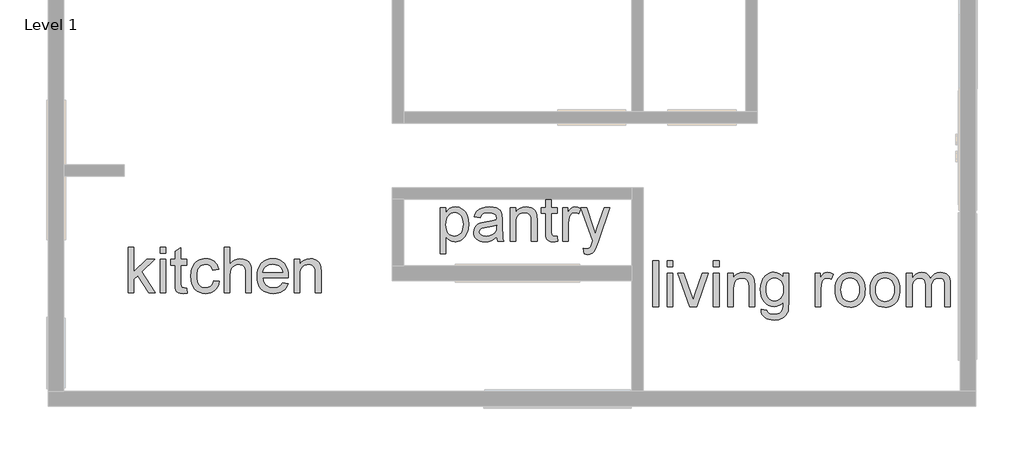
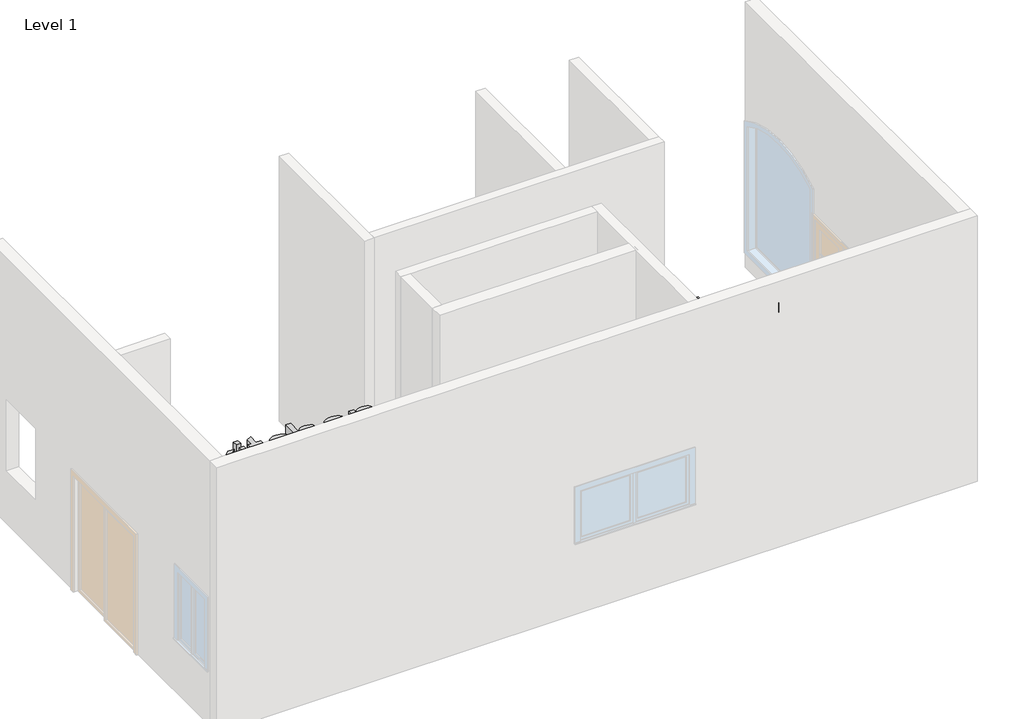
# One storey, part 2 of 3: 3 proxies.
"""IFC4 building model written with IfcOpenShell, lengths in millimetres."""

from ifc_helpers import new_model, si_unit, origin, origin_with_axes, place, context, project, spatial, polyline, outline, extrude, element, save

model = new_model("IFC4")

# Units and contexts
model_context = context("Model", 3, world=origin())
ifc_project = project(units=[si_unit("LENGTHUNIT", "METRE", prefix="MILLI")], contexts=[model_context])

# Site, building, storey
site = spatial("IfcSite", under=ifc_project)
building = spatial("IfcBuilding", under=site)
storey = spatial("IfcBuildingStorey", under=building, Name="Level 1", Elevation=0.0)

# Proxies
placement = place(None, origin())
element("IfcBuildingElementProxy", 1, Name="24\" Arial", ObjectType="24\" Arial", at=placement, inside=storey, context=model_context, shape_type="SweptSolid", body=[
    extrude(outline(polyline([(-2541.0046278, -2163.6481943), (-2541.0046278, -1554.5140062), (-2464.8628543, -1554.5140062), (-2464.8628543, -1881.8344036), (-2294.1387215, -1716.3152749), (-2188.8489253, -1716.3152749), (-2361.6550597, -1883.9164053), (-2179.3312036, -2163.6481943), (-2268.2624157, -2163.6481943), (-2416.2332451, -1936.8587322), (-2464.8628543, -1984.0011974), (-2464.8628543, -2163.6481943), (-2541.0046278, -2163.6481943)])), origin_with_axes(), (0.0, 0.0, 1.0), 152.4),
    extrude(outline(polyline([(-2112.7071518, -2163.6481943), (-2112.7071518, -1716.3152749), (-2036.5653783, -1716.3152749), (-2036.5653783, -2163.6481943), (-2112.7071518, -2163.6481943)])), origin_with_axes(), (0.0, 0.0, 1.0), 152.4),
    extrude(outline(polyline([(-2112.7071518, -1630.6557797), (-2112.7071518, -1554.5140062), (-2036.5653783, -1554.5140062), (-2036.5653783, -1630.6557797), (-2112.7071518, -1630.6557797)])), origin_with_axes(), (0.0, 0.0, 1.0), 152.4),
    extrude(outline(polyline([(-1760.5514493, -2100.1471449), (-1751.0337276, -2165.8789103), (-1781.1855725, -2171.3441646), (-1807.9913433, -2173.165916), (-1844.5379075, -2170.005735), (-1871.7898215, -2160.5251919), (-1891.0483365, -2145.9140019), (-1903.6147034, -2127.3618803), (-1910.5299231, -2095.4998198), (-1912.8349963, -2040.9588131), (-1912.8349963, -1792.4570484), (-1969.9413265, -1792.4570484), (-1969.9413265, -1716.3152749), (-1912.8349963, -1716.3152749), (-1912.8349963, -1607.6050475), (-1836.6932228, -1562.8420126), (-1836.6932228, -1716.3152749), (-1760.5514493, -1716.3152749), (-1760.5514493, -1792.4570484), (-1836.6932228, -1792.4570484), (-1836.6932228, -2038.7280971), (-1832.677934, -2077.9886991), (-1819.6654238, -2091.8934956), (-1808.6791474, -2095.7414808), (-1793.7147608, -2097.0241425), (-1760.5514493, -2100.1471449)])), origin_with_axes(), (0.0, 0.0, 1.0), 152.4),
    extrude(outline(polyline([(-1398.8780251, -2001.8469256), (-1322.7362516, -2011.3646473), (-1331.0177848, -2047.2931172), (-1343.9652324, -2079.0854678), (-1361.5785943, -2106.7416991), (-1383.8578705, -2130.2618112), (-1409.8643015, -2149.032357), (-1438.6591274, -2162.4398898), (-1470.2423484, -2170.4844094), (-1504.6139645, -2173.165916), (-1547.3182343, -2169.4248193), (-1585.6075453, -2158.2015293), (-1619.4818976, -2139.496046), (-1648.941291, -2113.3083694), (-1672.7867158, -2080.1311159), (-1689.8191621, -2040.456902), (-1700.0386299, -1994.2857277), (-1703.4451191, -1941.617593), (-1697.6266682, -1873.8595939), (-1690.3536045, -1843.3684943), (-1680.1713153, -1815.1359946), (-1667.0100908, -1789.7290686), (-1650.800221, -1767.7146899), (-1631.5417061, -1749.0928584), (-1609.2345459, -1733.8635742), (-1584.88721, -1722.02219), (-1559.5081679, -1713.5640585), (-1533.0974197, -1708.4891795), (-1505.6549653, -1706.7975532), (-1471.8735595, -1709.1212157), (-1441.3173974, -1716.0922033), (-1413.9864788, -1727.7105159), (-1389.8808038, -1743.9761535), (-1369.409337, -1764.5173302), (-1352.9810429, -1788.96226), (-1340.5959217, -1817.3109427), (-1332.2539732, -1849.5633785), (-1408.3957468, -1859.0811002), (-1422.2075968, -1825.8620208), (-1443.7154171, -1802.0491273), (-1471.7294925, -1787.7167769), (-1505.0601077, -1782.9393267), (-1530.9317662, -1785.2908732), (-1554.2659852, -1792.3455126), (-1575.0627648, -1804.103245), (-1593.3221049, -1820.5640703), (-1608.1888977, -1842.1090692), (-1618.8080354, -1869.1193223), (-1625.1795181, -1901.5948297), (-1627.3033456, -1939.5355914), (-1625.2259913, -1978.047974), (-1618.9939284, -2010.8999148), (-1608.607157, -2038.0914136), (-1594.0656769, -2059.6224705), (-1576.1688282, -2075.985702), (-1555.7159507, -2087.6737245), (-1532.7070444, -2094.686538), (-1507.1421093, -2097.0241425), (-1467.7142036, -2091.1871022), (-1450.663168, -2083.8908019), (-1435.3874106, -2073.6759814), (-1422.3144853, -2060.4311051), (-1411.8719459, -2044.044637), (-1404.0597925, -2024.5165771), (-1398.8780251, -2001.8469256)])), origin_with_axes(), (0.0, 0.0, 1.0), 152.4),
    extrude(outline(polyline([(-1256.1121997, -2163.6481943), (-1256.1121997, -1554.5140062), (-1179.9704262, -1554.5140062), (-1179.9704262, -1778.4778947), (-1152.0028241, -1747.1177453), (-1120.5962015, -1724.7176386), (-1085.7505583, -1711.2775745), (-1047.4658946, -1706.7975532), (-1001.4759659, -1711.6865391), (-961.9551138, -1726.353497), (-930.8366253, -1749.6458901), (-919.1532501, -1764.0944237), (-910.0537877, -1780.4111819), (-898.3425286, -1822.6832505), (-894.4387755, -1880.495974), (-894.4387755, -2163.6481943), (-970.580549, -2163.6481943), (-970.580549, -1888.3778373), (-972.095577, -1862.6688352), (-976.6406609, -1840.7148717), (-984.2158007, -1822.5159468), (-994.8209965, -1808.0720605), (-1008.2052926, -1797.0764895), (-1024.1177335, -1789.2225102), (-1042.5583193, -1784.5101226), (-1063.5270499, -1782.9393267), (-1095.7051285, -1787.1776871), (-1125.9127413, -1799.8927685), (-1150.9339393, -1819.8576769), (-1167.5527737, -1845.8455185), (-1176.8660131, -1880.3844382), (-1179.9704262, -1926.0025809), (-1179.9704262, -2163.6481943), (-1256.1121997, -2163.6481943)])), origin_with_axes(), (0.0, 0.0, 1.0), 152.4),
    extrude(outline(polyline([(-476.5513076, -2030.4000906), (-401.8966781, -2039.9178123), (-413.3430397, -2069.8187017), (-428.7953954, -2096.1690347), (-448.2537454, -2118.9688113), (-471.7180895, -2138.2180317), (-498.946767, -2153.507731), (-529.6981168, -2164.4289449), (-563.972139, -2170.9816732), (-601.7688336, -2173.165916), (-649.01354, -2169.3969354), (-691.1090102, -2158.0899935), (-728.0552443, -2139.2450905), (-759.8522423, -2112.8622262), (-785.4218246, -2079.6756781), (-803.6858121, -2040.4197234), (-814.6442045, -1995.0943623), (-818.297002, -1943.6995946), (-814.6070259, -1890.5620801), (-803.5370977, -1843.7263383), (-785.0872172, -1803.1923692), (-759.2573847, -1768.960173), (-727.5440386, -1741.7640268), (-691.4436176, -1722.3382081), (-650.9561218, -1710.6827169), (-606.0815512, -1706.7975532), (-562.6522987, -1710.6734223), (-523.3777547, -1722.3010295), (-488.2579194, -1741.680375), (-457.2927926, -1768.8114586), (-432.0159917, -1802.9692976), (-413.9611339, -1843.4289095), (-403.1282192, -1890.1902941), (-399.5172477, -1943.2534514), (-399.9633909, -1963.7760388), (-742.1552285, -1963.7760388), (-737.744917, -1994.1602499), (-728.9754147, -2020.7708331), (-715.8467214, -2043.6077884), (-698.3588373, -2062.6711157), (-677.4784059, -2077.7005649), (-654.1720708, -2088.4358858), (-628.439832, -2094.8770783), (-600.2816896, -2097.0241425), (-559.7570152, -2093.0460322), (-525.6270601, -2081.1117015), (-497.8918242, -2060.4775783), (-476.5513076, -2030.4000906)]), holes=[polyline([(-742.1552285, -1887.6342653), (-475.6590212, -1887.6342653), (-485.9574935, -1847.4070197), (-494.815295, -1831.5875253), (-506.1454735, -1818.630783), (-526.9097218, -1803.0157709), (-550.5367223, -1791.8621908), (-577.026475, -1785.1700427), (-606.37898, -1782.9393267), (-633.1522196, -1784.7192522), (-657.7040378, -1790.0590287), (-680.0344346, -1798.9586561), (-700.1434101, -1811.4181346), (-717.0178473, -1826.8611957), (-729.6446295, -1844.7115712), (-738.0237565, -1864.9692611), (-742.1552285, -1887.6342653)])]), origin_with_axes(), (0.0, 0.0, 1.0), 152.4),
    extrude(outline(polyline([(-323.3754741, -2163.6481943), (-323.3754741, -1716.3152749), (-247.2337006, -1716.3152749), (-247.2337006, -1778.7753235), (-220.7811265, -1747.285049), (-189.0120125, -1724.7919958), (-151.9263586, -1711.2961638), (-109.5241649, -1706.7975532), (-71.9923679, -1710.4224667), (-37.6207519, -1721.2972073), (-8.956051, -1738.0647561), (11.4550006, -1759.3680941), (25.3040292, -1785.1514534), (34.2826612, -1815.3590662), (38.2979501, -1888.9726949), (38.2979501, -2163.6481943), (-37.8438235, -2163.6481943), (-37.8438235, -1899.2339886), (-40.0373609, -1859.8618508), (-46.6179731, -1831.8663648), (-58.7567862, -1811.8085099), (-77.6249258, -1796.2492656), (-101.8096054, -1786.2668114), (-129.8980379, -1782.9393267), (-153.01848, -1784.8075514), (-174.493769, -1790.4122254), (-194.323905, -1799.7533487), (-212.5088879, -1812.8309214), (-227.7009935, -1831.1320874), (-238.5524974, -1856.1439908), (-245.0633998, -1887.8666315), (-247.2337006, -1926.3000097), (-247.2337006, -2163.6481943), (-323.3754741, -2163.6481943)])), origin_with_axes(), (0.0, 0.0, 1.0), 152.4),
])
element("IfcBuildingElementProxy", 2, Name="24\" Arial", ObjectType="24\" Arial", at=placement, inside=storey, context=model_context, shape_type="SweptSolid", body=[
    extrude(outline(polyline([(1631.9732742, -1642.5079695), (1631.9732742, -1023.8560597), (1708.1150477, -1023.8560597), (1708.1150477, -1098.5106892), (1732.9503528, -1061.6852856), (1760.7599458, -1035.3814258), (1793.1796853, -1019.59911), (1831.8454297, -1014.338338), (1858.400245, -1016.1786787), (1883.3377912, -1021.6997009), (1906.6580682, -1030.9014045), (1928.3610762, -1043.7837895), (1947.9727879, -1060.0122485), (1965.0191761, -1079.2521742), (1979.500241, -1101.5035665), (1991.4159824, -1126.7664255), (2007.3656019, -1182.8689334), (2012.6821418, -1244.1020882), (2006.6777978, -1309.2204067), (1999.1723679, -1339.2003005), (1988.664766, -1367.4606841), (1975.2990591, -1393.2626328), (1959.2193145, -1415.8672218), (1940.425532, -1435.2744512), (1918.9177117, -1451.4843209), (1895.7507964, -1464.2691121), (1871.9797288, -1473.4011058), (1847.6045089, -1478.8803021), (1822.6251368, -1480.7067008), (1787.6214846, -1475.8177149), (1756.372871, -1461.150757), (1729.622868, -1439.0109005), (1708.1150477, -1411.7032185), (1708.1150477, -1642.5079695), (1631.9732742, -1642.5079695)]), holes=[polyline([(1708.1150477, -1251.091665), (1710.1738127, -1287.7869436), (1716.3501077, -1319.3515753), (1726.6439327, -1345.7855601), (1741.0552876, -1367.0888981), (1758.403752, -1383.4846609), (1777.5089053, -1395.19592), (1798.3707474, -1402.2226755), (1820.9892784, -1404.5649273), (1843.9331221, -1402.1390236), (1865.1760449, -1394.8613126), (1884.7180467, -1382.7317942), (1902.5591275, -1365.7504685), (1917.4259204, -1343.6756746), (1928.0450581, -1316.2657514), (1934.4165407, -1283.5206992), (1936.5403683, -1245.4405178), (1934.4676613, -1209.0612573), (1928.2495404, -1177.5523935), (1917.8860055, -1150.9139264), (1903.3770568, -1129.1458559), (1885.9867664, -1112.2295927), (1866.979207, -1100.1465476), (1846.3543785, -1092.8967205), (1824.1122808, -1090.4801115), (1801.939893, -1093.0500823), (1781.0780509, -1100.7599945), (1761.5267544, -1113.6098483), (1743.2860036, -1131.5996435), (1727.8987104, -1154.4877193), (1716.9077867, -1182.0324149), (1710.3132325, -1214.2337301), (1708.1150477, -1251.091665)])]), origin_with_axes(), (0.0, 0.0, 1.0), 152.4),
    extrude(outline(polyline([(2383.8732877, -1414.082649), (2347.4940272, -1445.2754947), (2310.0365874, -1465.6865463), (2270.6458603, -1476.9516622), (2228.4667382, -1480.7067008), (2194.564502, -1478.4481008), (2164.8355637, -1471.6723009), (2139.2799233, -1460.3793011), (2117.8975808, -1444.5691013), (2101.0138489, -1425.2455237), (2088.9540404, -1403.4123907), (2081.7181553, -1379.0697021), (2079.3061936, -1352.217458), (2082.9496964, -1320.6528263), (2093.880205, -1291.9881254), (2110.7407002, -1267.4502492), (2132.1741633, -1248.2660914), (2157.362665, -1233.7664373), (2185.4882762, -1223.282072), (2251.368756, -1211.8310631), (2329.2207452, -1199.7851966), (2383.4271445, -1185.6573284), (2383.8732877, -1168.7038867), (2378.631105, -1134.7226459), (2372.0783767, -1122.1376897), (2362.9045571, -1112.4898429), (2347.047884, -1102.8605854), (2327.7336012, -1095.9825444), (2278.7322059, -1090.4801115), (2233.3743135, -1094.1422037), (2201.698146, -1105.1284801), (2180.0973792, -1125.4465852), (2164.9656888, -1157.1041633), (2088.8239153, -1147.5864417), (2102.0409077, -1105.9464093), (2121.7641552, -1073.229241), (2149.8339985, -1048.2080429), (2188.0907782, -1029.6559213), (2234.8800468, -1018.1677338), (2288.5473564, -1014.338338), (2340.0211286, -1017.7215906), (2380.8246425, -1027.8713485), (2411.5899342, -1043.133164), (2432.9490401, -1061.8525893), (2447.1140869, -1084.996268), (2456.2972012, -1113.5308437), (2460.0150612, -1180.1548956), (2460.0150612, -1274.8859693), (2463.8816356, -1407.1674293), (2469.6071401, -1439.8660083), (2479.0505046, -1471.1889791), (2402.9087311, -1471.1889791), (2390.7141501, -1444.7178157), (2383.8732877, -1414.082649)]), holes=[polyline([(2383.8732877, -1261.7991019), (2332.7155336, -1274.4770047), (2261.0351921, -1285.147263), (2195.5264983, -1297.4905583), (2178.48011, -1305.9301006), (2165.8579752, -1317.5670025), (2158.0504692, -1331.5089776), (2155.4479671, -1346.8637395), (2161.1177037, -1369.5055071), (2178.1269133, -1388.0576287), (2206.1038101, -1400.4381026), (2244.676608, -1404.5649273), (2285.5730684, -1400.0105487), (2321.7106679, -1386.3474131), (2351.007405, -1366.215201), (2371.381278, -1342.2535931), (2380.4156778, -1317.5670025), (2383.4271445, -1283.3626901), (2383.8732877, -1261.7991019)])]), origin_with_axes(), (0.0, 0.0, 1.0), 152.4),
    extrude(outline(polyline([(2564.7099998, -1471.1889791), (2564.7099998, -1023.8560597), (2640.8517733, -1023.8560597), (2640.8517733, -1086.3161083), (2667.3043475, -1054.8258338), (2699.0734615, -1032.3327806), (2736.1591153, -1018.8369486), (2778.561309, -1014.338338), (2816.0931061, -1017.9632515), (2850.4647221, -1028.8379921), (2879.1294229, -1045.6055409), (2899.5404745, -1066.9088789), (2913.3895032, -1092.6922382), (2922.3681352, -1122.899851), (2926.383424, -1196.5134797), (2926.383424, -1471.1889791), (2850.2416505, -1471.1889791), (2850.2416505, -1206.7747734), (2848.0481131, -1167.4026356), (2841.4675008, -1139.4071496), (2829.3286878, -1119.3492947), (2810.4605481, -1103.7900504), (2786.2758686, -1093.8075963), (2758.187436, -1090.4801115), (2735.0669939, -1092.3483362), (2713.5917049, -1097.9530102), (2693.7615689, -1107.2941335), (2675.576586, -1120.3717062), (2660.3844805, -1138.6728722), (2649.5329765, -1163.6847756), (2643.0220741, -1195.4074164), (2640.8517733, -1233.8407945), (2640.8517733, -1471.1889791), (2564.7099998, -1471.1889791)])), origin_with_axes(), (0.0, 0.0, 1.0), 152.4),
    extrude(outline(polyline([(3192.8796313, -1407.6879297), (3202.397353, -1473.4196951), (3172.2455081, -1478.8849494), (3145.4397373, -1480.7067008), (3108.8931731, -1477.5465198), (3081.6412591, -1468.0659767), (3062.3827441, -1453.4547867), (3049.8163772, -1434.9026652), (3042.9011575, -1403.0406047), (3040.5960843, -1348.499598), (3040.5960843, -1099.9978332), (2983.4897541, -1099.9978332), (2983.4897541, -1023.8560597), (3040.5960843, -1023.8560597), (3040.5960843, -915.1458323), (3116.7378578, -870.3827974), (3116.7378578, -1023.8560597), (3192.8796313, -1023.8560597), (3192.8796313, -1099.9978332), (3116.7378578, -1099.9978332), (3116.7378578, -1346.2688819), (3120.7531466, -1385.5294839), (3133.7656567, -1399.4342804), (3144.7519331, -1403.2822656), (3159.7163198, -1404.5649273), (3192.8796313, -1407.6879297)])), origin_with_axes(), (0.0, 0.0, 1.0), 152.4),
    extrude(outline(polyline([(3269.0214048, -1471.1889791), (3269.0214048, -1023.8560597), (3335.6454566, -1023.8560597), (3335.6454566, -1090.0339683), (3360.2576901, -1051.6656528), (3382.9366363, -1029.0610637), (3405.6899397, -1018.0190194), (3430.5252447, -1014.338338), (3468.4474171, -1020.2125569), (3506.9644471, -1037.8352134), (3481.5342844, -1106.0951237), (3454.7656922, -1094.3838646), (3427.9970999, -1090.4801115), (3405.2623858, -1094.2351502), (3384.9442807, -1105.5002661), (3368.5299287, -1123.4203514), (3357.5064737, -1147.1402985), (3348.2490022, -1189.6726173), (3345.1631783, -1236.0715105), (3345.1631783, -1471.1889791), (3269.0214048, -1471.1889791)])), origin_with_axes(), (0.0, 0.0, 1.0), 152.4),
    extrude(outline(polyline([(3554.5530555, -1642.5079695), (3545.0353338, -1569.1917696), (3583.7010782, -1575.8839177), (3604.0377726, -1573.7833268), (3619.8386777, -1567.481554), (3632.1447944, -1557.4247426), (3641.9971235, -1544.0590358), (3662.8171397, -1487.9937065), (3668.7657158, -1469.5531207), (3506.9644471, -1023.8560597), (3587.2702238, -1023.8560597), (3673.0784334, -1272.20911), (3702.9700281, -1371.5503302), (3732.8616228, -1283.8088333), (3821.0492628, -1023.8560597), (3900.760182, -1023.8560597), (3745.0562037, -1481.896416), (3704.6058865, -1581.2376361), (3683.8974061, -1612.9509822), (3660.4377093, -1634.923535), (3633.1857952, -1647.7501522), (3601.1006631, -1652.0256912), (3579.0537531, -1649.6462608), (3554.5530555, -1642.5079695)])), origin_with_axes(), (0.0, 0.0, 1.0), 152.4),
])
element("IfcBuildingElementProxy", 3, Name="24\" Arial", ObjectType="24\" Arial", at=placement, inside=storey, context=model_context, shape_type="SweptSolid", body=[
    extrude(outline(polyline([(4474.7005786, -2345.8743036), (4474.7005786, -1736.7401154), (4550.8423522, -1736.7401154), (4550.8423522, -2345.8743036), (4474.7005786, -2345.8743036)])), origin_with_axes(), (0.0, 0.0, 1.0), 152.4),
    extrude(outline(polyline([(4665.0550124, -2345.8743036), (4665.0550124, -1898.5413841), (4741.196786, -1898.5413841), (4741.196786, -2345.8743036), (4665.0550124, -2345.8743036)])), origin_with_axes(), (0.0, 0.0, 1.0), 152.4),
    extrude(outline(polyline([(4665.0550124, -1812.8818889), (4665.0550124, -1736.7401154), (4741.196786, -1736.7401154), (4741.196786, -1812.8818889), (4665.0550124, -1812.8818889)])), origin_with_axes(), (0.0, 0.0, 1.0), 152.4),
    extrude(outline(polyline([(4965.1606745, -2345.8743036), (4807.8208378, -1898.5413841), (4888.4240433, -1898.5413841), (4983.7499746, -2166.5247355), (5012.4518541, -2256.6456627), (5040.558876, -2171.5810251), (5136.4796649, -1898.5413841), (5217.0828704, -1898.5413841), (5061.676321, -2345.8743036), (4965.1606745, -2345.8743036)])), origin_with_axes(), (0.0, 0.0, 1.0), 152.4),
    extrude(outline(polyline([(5283.7069223, -2345.8743036), (5283.7069223, -1898.5413841), (5359.8486958, -1898.5413841), (5359.8486958, -2345.8743036), (5283.7069223, -2345.8743036)])), origin_with_axes(), (0.0, 0.0, 1.0), 152.4),
    extrude(outline(polyline([(5283.7069223, -1812.8818889), (5283.7069223, -1736.7401154), (5359.8486958, -1736.7401154), (5359.8486958, -1812.8818889), (5283.7069223, -1812.8818889)])), origin_with_axes(), (0.0, 0.0, 1.0), 152.4),
    extrude(outline(polyline([(5474.0613561, -2345.8743036), (5474.0613561, -1898.5413841), (5550.2031296, -1898.5413841), (5550.2031296, -1961.0014327), (5576.6557037, -1929.5111582), (5608.4248177, -1907.018105), (5645.5104716, -1893.5222731), (5687.9126653, -1889.0236624), (5725.4444623, -1892.648576), (5759.8160783, -1903.5233166), (5788.4807792, -1920.2908653), (5808.8918308, -1941.5942033), (5822.7408594, -1967.3775627), (5831.7194914, -1997.5851755), (5835.7347803, -2071.1988042), (5835.7347803, -2345.8743036), (5759.5930067, -2345.8743036), (5759.5930067, -2081.4600979), (5757.3994693, -2042.0879601), (5750.8188571, -2014.092474), (5738.680044, -1994.0346191), (5719.8119044, -1978.4753749), (5695.6272248, -1968.4929207), (5667.5387923, -1965.165436), (5644.4183502, -1967.0336606), (5622.9430612, -1972.6383346), (5603.1129252, -1981.979458), (5584.9279423, -1995.0570306), (5569.7358367, -2013.3581967), (5558.8843328, -2038.3701001), (5552.3734304, -2070.0927408), (5550.2031296, -2108.5261189), (5550.2031296, -2345.8743036), (5474.0613561, -2345.8743036)])), origin_with_axes(), (0.0, 0.0, 1.0), 152.4),
    extrude(outline(polyline([(5921.3942755, -2383.9451903), (5997.536049, -2393.462912), (6005.9384127, -2417.2572162), (6022.2226396, -2433.6158004), (6054.2334145, -2446.3308817), (6096.1336971, -2450.5692421), (6140.8223747, -2445.7732027), (6158.8725852, -2439.7781534), (6174.0600434, -2431.3850844), (6197.1107757, -2408.3343521), (6211.2386438, -2377.550471), (6215.3654684, -2344.7961241), (6216.4436478, -2288.7679734), (6191.1064317, -2313.7519928), (6162.8321061, -2331.597721), (6131.6206711, -2342.3051579), (6097.4721267, -2345.8743036), (6055.7252059, -2341.719595), (6018.9695121, -2329.2554692), (5987.2050454, -2308.4819262), (5960.4318058, -2279.3989661), (5939.1888831, -2244.5068497), (5924.0153668, -2206.3058378), (5914.911257, -2164.7959305), (5911.8765538, -2119.9771278), (5917.3232187, -2058.5023121), (5933.6632136, -2001.9722503), (5945.7741426, -1976.4816724), (5960.32027, -1954.0676238), (5977.3015957, -1934.7301043), (5996.7181198, -1918.4691139), (6018.2584714, -1905.5867289), (6041.6112797, -1896.3850253), (6066.7765448, -1890.8640032), (6093.7542667, -1889.0236624), (6129.3620712, -1893.1876657), (6161.6795695, -1905.6796754), (6190.7067618, -1926.4996916), (6216.4436478, -1955.6477143), (6216.4436478, -1898.5413841), (6292.5854214, -1898.5413841), (6292.5854214, -2284.7526846), (6287.3804173, -2373.9255575), (6280.8741623, -2407.0935164), (6271.7654052, -2432.6491568), (6259.8357218, -2453.2600433), (6244.8666878, -2471.5937406), (6226.8583033, -2487.6502487), (6205.8105681, -2501.4295674), (6181.9372594, -2512.490201), (6155.452154, -2520.3906536), (6126.3552519, -2525.1309251), (6094.6465531, -2526.7110157), (6057.342475, -2524.484947), (6023.8027301, -2517.8067409), (5994.0273186, -2506.6763974), (5968.0162403, -2491.0939165), (5947.0056838, -2471.040709), (5932.2318375, -2446.4981854), (5923.6947014, -2417.4663458), (5921.3942755, -2383.9451903)]), holes=[polyline([(5988.0183273, -2114.7721238), (5990.0492083, -2152.420104), (5996.1418515, -2184.6121245), (6006.2962567, -2211.3481855), (6020.512424, -2232.6282869), (6037.7958258, -2248.8613933), (6057.1519346, -2260.4564692), (6078.5807504, -2267.4135148), (6102.0822732, -2269.73253), (6125.3514297, -2267.4274568), (6146.6780043, -2260.5122371), (6166.061997, -2248.986871), (6183.5034079, -2232.8513585), (6197.9147629, -2211.7803867), (6208.2085879, -2185.448643), (6214.3848829, -2153.8561274), (6216.4436478, -2117.0028398), (6214.3244676, -2081.6878168), (6207.966927, -2050.9922349), (6197.3710259, -2024.9160941), (6182.5367643, -2003.4593943), (6164.7189201, -1986.7057875), (6145.172271, -1974.7389256), (6123.8968169, -1967.5588084), (6100.892558, -1965.165436), (6078.274027, -1967.5216298), (6057.4121848, -1974.5902112), (6038.3070316, -1986.3711801), (6020.9585672, -2002.8645367), (6006.5472122, -2023.9959237), (5996.2533873, -2049.6909839), (5990.0770923, -2079.9497172), (5988.0183273, -2114.7721238)])]), origin_with_axes(), (0.0, 0.0, 1.0), 152.4),
    extrude(outline(polyline([(6644.7411239, -2345.8743036), (6644.7411239, -1898.5413841), (6711.3651757, -1898.5413841), (6711.3651757, -1964.7192928), (6735.9774091, -1926.3509772), (6758.6563554, -1903.7463882), (6781.4096588, -1892.7043439), (6806.2449638, -1889.0236624), (6844.1671362, -1894.8978813), (6882.6841661, -1912.5205379), (6857.2540035, -1980.7804481), (6830.4854112, -1969.069189), (6803.716819, -1965.165436), (6780.9821049, -1968.9204746), (6760.6639998, -1980.1855905), (6744.2496477, -1998.1056759), (6733.2261927, -2021.8256229), (6723.9687212, -2064.3579417), (6720.8828974, -2110.7568349), (6720.8828974, -2345.8743036), (6644.7411239, -2345.8743036)])), origin_with_axes(), (0.0, 0.0, 1.0), 152.4),
    extrude(outline(polyline([(6911.2373312, -2122.2078438), (6915.3548612, -2064.2742898), (6927.7074511, -2014.3527242), (6948.2951011, -1972.443147), (6977.117811, -1938.5455581), (7006.1357086, -1916.8797288), (7038.1650728, -1901.4041364), (7073.2059036, -1892.1187809), (7111.2582011, -1889.0236624), (7153.2653721, -1892.7926431), (7191.2479597, -1904.0995849), (7225.2059638, -1922.9444879), (7255.1393844, -1949.3273522), (7279.5703722, -1982.3558913), (7297.0210777, -2021.1378188), (7307.491501, -2065.6731347), (7310.9816422, -2115.961839), (7309.4387302, -2156.7188796), (7304.8099945, -2192.8843631), (7297.0954349, -2224.4582895), (7286.2950515, -2251.4406587), (7272.5436167, -2274.7469938), (7255.9759029, -2295.2928178), (7236.5919102, -2313.0781307), (7214.3916384, -2328.1029326), (7190.2394902, -2340.0419106), (7164.9998679, -2348.5697521), (7138.6727715, -2353.6864569), (7111.2582011, -2355.3920252), (7068.6375831, -2351.6369866), (7030.3017988, -2340.3718707), (6996.2508482, -2321.5966775), (6966.4847313, -2295.3114071), (6942.3139938, -2261.9622026), (6925.0491812, -2221.9952072), (6914.6902937, -2175.4104209), (6911.2373312, -2122.2078438)]), holes=[polyline([(6987.3791047, -2122.0591294), (6989.5819368, -2158.9914216), (6996.190433, -2190.9696652), (7007.2045933, -2217.9938603), (7022.6244178, -2240.064007), (7041.3810217, -2257.207989), (7062.4055202, -2269.4536905), (7085.6979133, -2276.8011114), (7111.2582011, -2279.2502517), (7136.6883637, -2276.7871694), (7159.8878103, -2269.3979226), (7180.8565409, -2257.0825113), (7199.5945555, -2239.8409354), (7215.01438, -2217.5523644), (7226.0285404, -2190.0959681), (7232.6370366, -2157.4717463), (7234.8398686, -2119.679699), (7232.6230946, -2083.9185328), (7225.9727725, -2052.7768077), (7214.8889022, -2026.2545237), (7199.3714839, -2004.3516807), (7180.5637595, -1987.2076986), (7159.6089708, -1974.9619972), (7136.507118, -1967.6145763), (7111.2582011, -1965.165436), (7085.6979133, -1967.6052816), (7062.4055202, -1974.9248186), (7041.3810217, -1987.1240468), (7022.6244178, -2004.2029663), (7007.2045933, -2026.2080504), (6996.190433, -2053.1857723), (6989.5819368, -2085.136132), (6987.3791047, -2122.0591294)])]), origin_with_axes(), (0.0, 0.0, 1.0), 152.4),
    extrude(outline(polyline([(7377.605694, -2122.2078438), (7381.723224, -2064.2742898), (7394.0758139, -2014.3527242), (7414.6634639, -1972.443147), (7443.4861738, -1938.5455581), (7472.5040714, -1916.8797288), (7504.5334356, -1901.4041364), (7539.5742664, -1892.1187809), (7577.6265639, -1889.0236624), (7619.6337349, -1892.7926431), (7657.6163225, -1904.0995849), (7691.5743266, -1922.9444879), (7721.5077472, -1949.3273522), (7745.938735, -1982.3558913), (7763.3894405, -2021.1378188), (7773.8598638, -2065.6731347), (7777.3500049, -2115.961839), (7775.807093, -2156.7188796), (7771.1783573, -2192.8843631), (7763.4637977, -2224.4582895), (7752.6634143, -2251.4406587), (7738.9119795, -2274.7469938), (7722.3442657, -2295.2928178), (7702.960273, -2313.0781307), (7680.7600012, -2328.1029326), (7656.607853, -2340.0419106), (7631.3682307, -2348.5697521), (7605.0411343, -2353.6864569), (7577.6265639, -2355.3920252), (7535.0059459, -2351.6369866), (7496.6701616, -2340.3718707), (7462.619211, -2321.5966775), (7432.8530941, -2295.3114071), (7408.6823565, -2261.9622026), (7391.417544, -2221.9952072), (7381.0586565, -2175.4104209), (7377.605694, -2122.2078438)]), holes=[polyline([(7453.7474675, -2122.0591294), (7455.9502996, -2158.9914216), (7462.5587958, -2190.9696652), (7473.5729561, -2217.9938603), (7488.9927806, -2240.064007), (7507.7493845, -2257.207989), (7528.773883, -2269.4536905), (7552.0662761, -2276.8011114), (7577.6265639, -2279.2502517), (7603.0567265, -2276.7871694), (7626.2561731, -2269.3979226), (7647.2249037, -2257.0825113), (7665.9629183, -2239.8409354), (7681.3827428, -2217.5523644), (7692.3969031, -2190.0959681), (7699.0053994, -2157.4717463), (7701.2082314, -2119.679699), (7698.9914574, -2083.9185328), (7692.3411352, -2052.7768077), (7681.257265, -2026.2545237), (7665.7398467, -2004.3516807), (7646.9321222, -1987.2076986), (7625.9773336, -1974.9619972), (7602.8754808, -1967.6145763), (7577.6265639, -1965.165436), (7552.0662761, -1967.6052816), (7528.773883, -1974.9248186), (7507.7493845, -1987.1240468), (7488.9927806, -2004.2029663), (7473.5729561, -2026.2080504), (7462.5587958, -2053.1857723), (7455.9502996, -2085.136132), (7453.7474675, -2122.0591294)])]), origin_with_axes(), (0.0, 0.0, 1.0), 152.4),
    extrude(outline(polyline([(7863.0095002, -2345.8743036), (7863.0095002, -1898.5413841), (7939.1512737, -1898.5413841), (7939.1512737, -1972.1550128), (7962.0532915, -1938.3410758), (7991.498743, -1911.8513231), (8026.4838059, -1894.7305776), (8066.0046581, -1889.0236624), (8108.3510839, -1894.8421134), (8126.3734104, -1902.1151771), (8142.295146, -1912.2974663), (8156.0698174, -1925.1008468), (8167.6509514, -1940.2371844), (8184.2326072, -1977.5087313), (8211.9864323, -1938.7965137), (8243.6440105, -1911.1449297), (8279.2053418, -1894.5539793), (8318.670426, -1889.0236624), (8349.152231, -1891.3240883), (8375.9068813, -1898.225366), (8398.9343769, -1909.7274955), (8418.2347178, -1925.8304768), (8433.4918859, -1946.7202029), (8444.3898631, -1972.5825667), (8450.9286495, -2003.4175684), (8453.1082449, -2039.2252079), (8453.1082449, -2345.8743036), (8376.9664714, -2345.8743036), (8376.9664714, -2071.9423762), (8375.2004879, -2033.9644359), (8369.9025373, -2008.3669696), (8359.975851, -1990.8372595), (8344.3236603, -1977.0625881), (8324.1914482, -1968.139724), (8300.8246979, -1965.165436), (8279.2471677, -1967.0708392), (8259.5750408, -1972.787049), (8241.8083171, -1982.3140654), (8225.9469968, -1995.6518883), (8212.9019554, -2013.190893), (8203.5840687, -2035.3214548), (8197.9933366, -2062.0435738), (8196.1297593, -2093.35725), (8196.1297593, -2345.8743036), (8119.9879858, -2345.8743036), (8119.9879858, -2063.4656553), (8115.5823216, -2020.4128361), (8110.0752415, -2003.5151622), (8102.3653292, -1989.7033122), (8092.1458614, -1978.9679913), (8079.1101147, -1971.299905), (8063.258089, -1966.6990532), (8044.5897843, -1965.165436), (8015.2558686, -1969.255082), (7988.2270261, -1981.5240201), (7965.9198659, -2001.6748215), (7950.750997, -2029.4100574), (7942.0512045, -2067.8899087), (7939.1512737, -2120.2745566), (7939.1512737, -2345.8743036), (7863.0095002, -2345.8743036)])), origin_with_axes(), (0.0, 0.0, 1.0), 152.4),
])

save(model, "model.ifc")

# Revit data of these elements
# Project information
#   Project Issue Date = "Issue Date"
#   Project Status = "Project  Status"
#   Client Name = "Owner"
#   Project Address = "## Street\nCity, State  Zip"
#   Project Name = "Project Name"
#   Project Number = "0001"
# Elements 1, 2, 3 (IfcBuildingElementProxy, "24\" Arial")
#   Phase Created = New Construction
